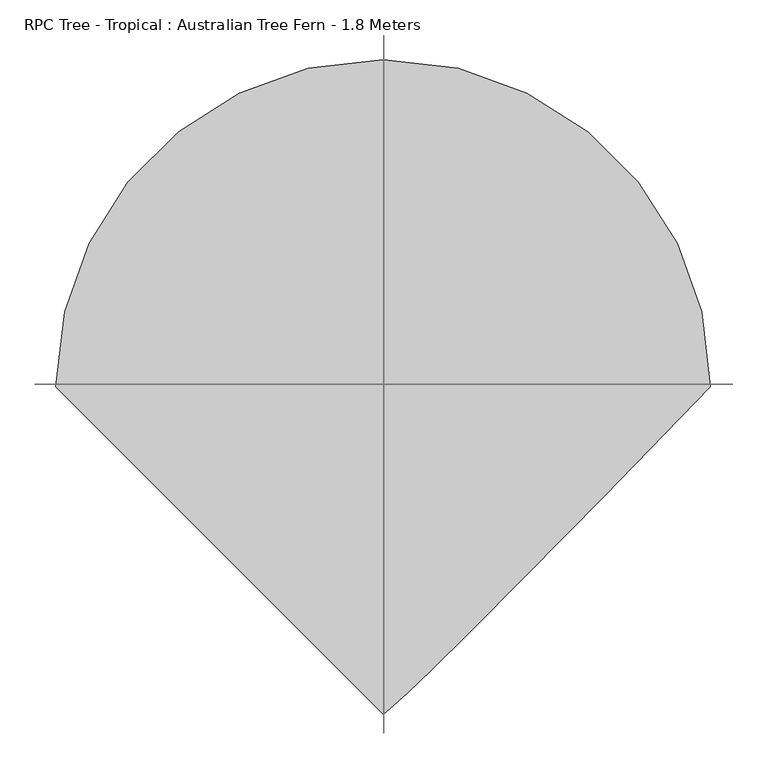
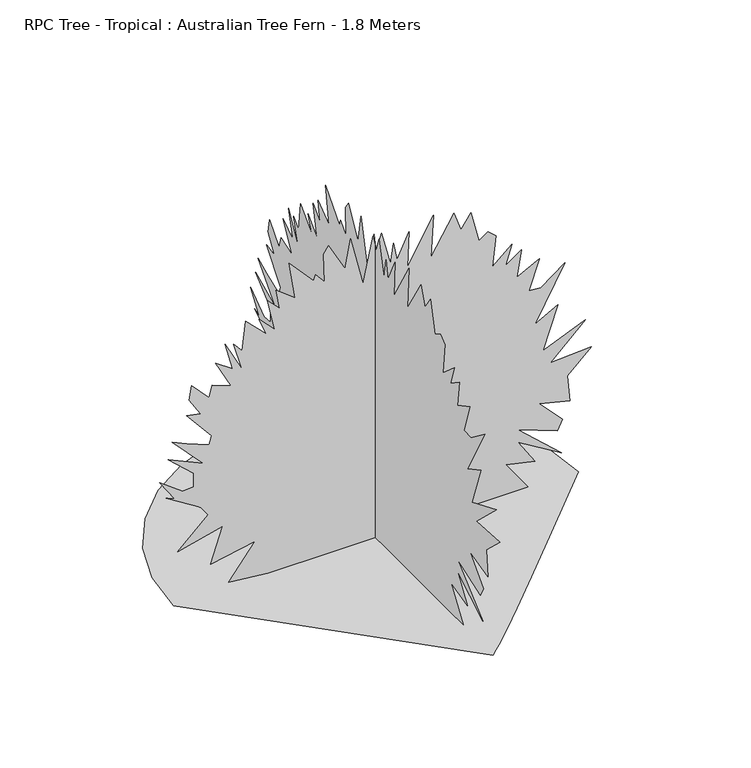
"""IFC4 building model written with IfcOpenShell, lengths in millimetres: geographic element geometry, RPC Tree - Tropical : Australian Tree Fern - 1.8 Meters."""

from ifc_helpers import new_model, si_unit, origin, place, context, project, spatial, triangles, source, transform, mapped, element, save


def rpc_tree_tropical_australian_tree_fern_1_8_meters_894294f9(model_context):
    return source(origin(), model_context, "Body", "Tessellation", [
        triangles([(-1121.4844528, 0.0, 0.0002091), (-1091.8312483, 257.014581, 0.0002091), (-1007.379063, 493.0422163, 0.0002091), (-874.8874409, 701.3197649, 0.0002091), (-701.1231199, 875.0840858, 0.0002091), (-492.845535, 1007.575708, 0.0002091), (-256.8179179, 1092.0278933, 0.0002091), (0.1967201, 1121.6810978, 0.0002091), (257.2112442, 1092.0278933, 0.0002091), (493.2388976, 1007.575708, 0.0002091), (701.5164099, 875.0840858, 0.0002091), (875.2807308, 701.3197649, 0.0002091), (1007.772353, 493.0422163, 0.0002091), (1092.2245382, 257.014581, 0.0002091), (1121.8777428, -9.81e-05, 0.0002091), (757.3559521, -373.9099531, 0.0002091), (487.118886, -649.203978, 0.0002091), (295.4501165, -842.3164639, 0.0002091), (166.6377574, -969.6837622, 0.0002091), (84.9673791, -1047.7439684, 0.0002091), (34.7249062, -1092.9297277, 0.0002091), (0.196524, -1121.6810978, 0.0002091), (-584.7020648, 9.9524755, 0.0280128), (-811.2515722, 9.9524573, 23.5990138), (-664.9373926, 9.9524755, 212.3913055), (-910.368124, 9.9524755, 165.1928965), (-844.2910526, 9.9524755, 363.42491), (-1094.439374, 9.9524755, 302.0672271), (-924.5263441, 9.9524948, 457.820202), (-967.0045652, 9.9524948, 519.177903), (-1155.7970387, 9.9524948, 637.1720089), (-1108.5994108, 9.9524948, 618.292638), (-1193.5540363, 9.9524948, 741.0079674), (-1066.121117, 9.9524948, 646.6127117), (-1004.7634523, 9.9524948, 651.3321184), (-1004.7634523, 9.9524948, 731.5673372), (-1146.3564085, 9.952513, 859.002146), (-952.8445284, 9.952513, 769.3262243), (-1122.7575583, 9.952513, 953.399291), (-1042.5223394, 9.952513, 915.6404039), (-919.8069374, 9.952513, 868.4427761), (-905.6469006, 9.952513, 915.6404039), (-1042.5223394, 9.952513, 1080.8322104), (-967.0045652, 9.952513, 1066.6740629), (-1028.3623026, 9.9525323, 1165.7887253), (-1014.2022657, 9.9525323, 1246.0258335), (-919.8069374, 9.9525323, 1142.1899477), (-900.9274939, 9.9525323, 1208.2670191), (-797.0915354, 9.9525323, 1170.508132), (-882.0480503, 9.9525323, 1330.9824211), (-787.652722, 9.9525323, 1264.9053497), (-830.1310158, 9.9525504, 1425.3776768), (-735.7356874, 9.9525323, 1246.0258335), (-782.9333879, 9.9525504, 1406.4983059), (-735.7356874, 9.9525323, 1354.5812714), (-716.8562439, 9.9525504, 1519.7729324), (-603.5815084, 9.9525504, 1406.4983059), (-641.3385424, 9.9525504, 1505.614785), (-556.3819911, 9.9525504, 1415.9388634), (-594.1408419, 9.9525504, 1595.2907066), (-528.0637705, 9.9525504, 1529.2136353), (-546.943214, 9.9525504, 1642.4884071), (-443.1072556, 9.9525504, 1562.2512989), (-476.146736, 9.9525697, 1774.6425499), (-339.2712971, 9.9525504, 1623.6088909), (-329.83252, 9.9525504, 1656.648444), (-279.7754919, 9.9525504, 1596.614463), (-284.4967516, 9.9525697, 1761.8062695), (-256.1691566, 9.9525697, 1800.0058273), (-164.5496218, 9.9525697, 1634.348933), (-134.8663864, 9.9525323, 1797.6189091), (-66.8546674, 9.9525323, 1511.5436382), (-8.8864392, 9.9525697, 1769.9232159), (9.9927528, 9.9525504, 1680.2472942), (38.3116059, 9.9525697, 1769.9232159), (85.5096334, 9.9525504, 1576.4113358), (104.3886955, 9.9525504, 1689.6861076), (123.2679392, 9.9525504, 1585.8501492), (189.3454011, 9.9525697, 1727.4448494), (179.9054977, 9.9525504, 1524.4943012), (326.2189688, 9.9525697, 1774.6425499), (312.0589319, 9.9525504, 1533.9331146), (439.4937043, 9.9525697, 1746.3243656), (477.2525914, 9.9525504, 1637.7690731), (533.8908857, 9.9525697, 1718.0042919), (576.3691432, 9.9525504, 1538.6524487), (628.2861414, 9.9525504, 1571.6918564), (670.7644352, 9.9525504, 1533.9331146), (651.8849916, 9.9525323, 1359.3006054), (760.4403568, 9.9525504, 1453.6958611), (722.6814697, 9.9525323, 1340.4212345), (812.3573914, 9.9525504, 1401.7788265), (788.7585411, 9.9525323, 1250.7453129), (911.4739431, 9.9525323, 1316.8223843), (854.8356125, 9.9525323, 1146.9092817), (920.9127565, 9.9525323, 1142.1899477), (1053.0668993, 9.9525323, 1241.3064995), (887.8750929, 9.952513, 939.2392542), (1015.3099016, 9.952513, 1010.0357323), (930.3533867, 9.952513, 769.3262243), (1166.3416712, 9.952513, 868.4427761), (972.8316078, 9.9524948, 684.3697094), (1199.3811516, 9.9524948, 698.5297462), (1067.2269361, 9.9524948, 575.8143442), (1081.386973, 9.9524755, 424.7807216), (911.4739431, 9.9524948, 467.2590154), (1038.9087519, 9.9524755, 330.3854296), (1010.5886055, 9.9524755, 273.7490065), (793.4779478, 9.9524755, 353.9842435), (1034.1874557, 9.9524755, 136.8741308), (793.4779478, 9.9524755, 283.1877836), (887.8750929, 9.9524755, 136.8741308), (727.4008764, 9.9524755, 174.6324366), (850.2137289, 9.9524755, 0.0285496), (14.7125365, 9.9524573, 9.11e-05), (2.9132547, 597.5662868, 0.0279397), (2.913236, 824.1176474, 23.5990138), (2.9132547, 677.8033951, 212.3913055), (2.9132547, 923.2323097, 165.1928965), (2.9132547, 857.1552383, 363.42491), (2.9132547, 1107.3054491, 302.0672271), (2.9132547, 937.3923466, 457.820202), (2.9132547, 979.8706404, 519.177903), (2.9132735, 1168.6612244, 637.1720089), (2.9132735, 1121.4635965, 618.292638), (2.9132735, 1206.4201115, 741.0079674), (2.9132735, 1078.9853027, 646.6127117), (2.9132735, 1017.6295275, 651.3321184), (2.9132735, 1017.6295275, 731.5673372), (2.9132735, 1159.2224836, 859.002146), (2.9132735, 965.7106035, 769.3262243), (2.9132735, 1135.6236334, 953.399291), (2.9132735, 1055.3865252, 915.6404039), (2.9132735, 932.6730125, 868.4427761), (2.9132735, 918.5129757, 915.6404039), (2.9132735, 1055.3865252, 1080.8322104), (2.9132735, 979.8706404, 1066.6740629), (2.9132735, 1041.2283051, 1165.7887253), (2.9132922, 1027.0682682, 1246.0258335), (2.9132735, 932.6730125, 1142.1899477), (2.9132735, 913.793569, 1208.2670191), (2.9132735, 809.9576105, 1170.5100214), (2.9132922, 894.9141254, 1330.9824211), (2.9132735, 800.5187971, 1264.9053497), (2.9132922, 842.9970909, 1425.3776768), (2.9132735, 748.5998732, 1246.0258335), (2.9132922, 795.7975737, 1406.4983059), (2.9132735, 748.5998732, 1354.5812714), (2.9132922, 729.722319, 1519.7729324), (2.9132735, 616.4457304, 1406.4983059), (2.9132922, 654.2046175, 1505.614785), (2.9132735, 569.2480662, 1415.9388634), (2.9132922, 607.0069533, 1595.2907066), (2.9132922, 540.9298456, 1529.2136353), (2.9132922, 559.8092892, 1642.4884071), (2.9132922, 455.9733307, 1562.2512989), (2.9132922, 489.010958, 1774.6425499), (2.9132922, 352.1373722, 1623.6088909), (2.9132922, 342.6985951, 1656.648444), (2.9132922, 292.641567, 1596.614463), (2.9132922, 297.3609555, 1761.8062695), (2.9132922, 269.0352317, 1800.0058273), (2.9132922, 177.4153154, 1634.348933), (2.9132547, 147.7320982, 1797.6189091), (2.9132547, 79.72057, 1511.5455276), (2.9132922, 21.7521334, 1769.9232159), (2.9132735, 2.872978, 1680.2472942), (2.9132922, -25.4458941, 1769.9232159), (2.9132735, -72.6439216, 1576.4113358), (2.9132735, -91.5229837, 1689.6861076), (2.9132735, -110.4020457, 1585.8518932), (2.9132735, -176.4793078, 1727.4448494), (2.9132735, -167.0397859, 1524.4943012), (2.9132735, -313.3528936, 1774.6425499), (2.9132735, -299.1947099, 1533.9331146), (2.9132735, -426.6276292, 1746.3243656), (2.9132735, -464.3864799, 1637.7690731), (2.9132735, -521.0248106, 1718.0061813), (2.9132735, -563.5030681, 1538.6524487), (2.9132735, -615.4200663, 1571.6918564), (2.9132735, -657.8983601, 1533.9331146), (2.9132547, -639.0189165, 1359.3006054), (2.9132547, -747.5742817, 1453.6958611), (2.9132547, -709.8153946, 1340.4212345), (2.9132547, -799.4913162, 1401.7788265), (2.9132547, -775.892466, 1250.7453129), (2.9132547, -898.607868, 1316.8223843), (2.9132547, -841.96961, 1146.9092817), (2.9132547, -908.0466814, 1142.1899477), (2.9132547, -1040.2008242, 1241.3064995), (2.9132547, -875.0090904, 939.2392542), (2.9132547, -1002.4438265, 1010.0357323), (2.913236, -917.4873116, 769.3262243), (2.913236, -1153.4774855, 868.4427761), (2.913236, -959.9656054, 684.3697094), (2.913236, -1186.5150764, 698.5297462), (2.913236, -1054.360861, 575.8143442), (2.913236, -1068.5208979, 424.7807216), (2.913236, -898.607868, 467.2590154), (2.9132173, -1026.0426767, 330.3854296), (2.9132173, -997.7244198, 273.7490065), (2.913236, -780.6137621, 353.9842435), (2.9132173, -1021.32327, 136.8739401), (2.913236, -780.6137621, 283.1877836), (2.9132173, -875.0090904, 136.8739401), (2.9132173, -714.5366907, 174.6324366), (2.913236, -837.3476538, 0.0284335), (2.913236, -1.8467684, 0.0)], [[22, 21, 1], [21, 20, 1], [20, 19, 1], [19, 18, 1], [18, 17, 1], [1, 17, 2], [2, 17, 3], [3, 17, 4], [17, 16, 4], [4, 16, 5], [5, 16, 6], [6, 16, 7], [7, 16, 8], [8, 16, 9], [9, 16, 10], [10, 16, 11], [11, 16, 12], [16, 15, 12], [15, 14, 12], [14, 13, 12], [31, 30, 32], [110, 109, 111], [52, 51, 53], [37, 36, 38], [33, 32, 34], [77, 76, 78], [101, 100, 102], [39, 38, 40], [79, 78, 80], [58, 57, 59], [71, 70, 72], [97, 96, 98], [73, 72, 74], [54, 53, 55], [81, 80, 82], [50, 49, 51], [28, 27, 29], [90, 89, 91], [75, 74, 76], [60, 59, 61], [64, 63, 65], [40, 38, 41], [103, 102, 104], [43, 42, 44], [99, 98, 100], [62, 61, 63], [94, 93, 95], [112, 111, 113], [92, 91, 93], [85, 84, 86], [83, 82, 84], [56, 55, 57], [46, 45, 47], [45, 44, 47], [114, 113, 115], [66, 65, 67], [24, 23, 25], [74, 72, 76], [26, 25, 27], [69, 68, 70], [68, 67, 70], [32, 30, 34], [34, 30, 35], [105, 104, 106], [51, 49, 53], [104, 102, 106], [96, 95, 98], [48, 47, 49], [108, 107, 109], [107, 106, 109], [84, 82, 86], [87, 86, 88], [88, 86, 89], [70, 67, 72], [23, 115, 25], [55, 53, 57], [86, 82, 89], [78, 76, 80], [65, 63, 67], [61, 59, 63], [44, 42, 47], [47, 42, 49], [36, 35, 38], [76, 72, 80], [113, 111, 115], [111, 109, 115], [102, 100, 106], [106, 100, 109], [109, 100, 115], [100, 98, 115], [115, 98, 25], [98, 95, 25], [95, 93, 25], [93, 91, 25], [91, 89, 25], [89, 82, 25], [82, 80, 25], [80, 72, 25], [25, 72, 27], [27, 72, 29], [72, 67, 29], [67, 63, 29], [63, 59, 29], [29, 59, 30], [30, 59, 35], [35, 59, 38], [38, 59, 41], [41, 59, 42], [42, 59, 49], [49, 59, 53], [53, 59, 57], [124, 123, 125], [203, 202, 204], [145, 144, 146], [130, 129, 131], [126, 125, 127], [170, 169, 171], [194, 193, 195], [132, 131, 133], [172, 171, 173], [151, 150, 152], [164, 163, 165], [190, 189, 191], [166, 165, 167], [147, 146, 148], [174, 173, 175], [143, 142, 144], [121, 120, 122], [183, 182, 184], [168, 167, 169], [153, 152, 154], [157, 156, 158], [133, 131, 134], [196, 195, 197], [136, 135, 137], [192, 191, 193], [155, 154, 156], [187, 186, 188], [205, 204, 206], [185, 184, 186], [178, 177, 179], [176, 175, 177], [149, 148, 150], [139, 138, 140], [138, 137, 140], [207, 206, 208], [159, 158, 160], [117, 116, 118], [167, 165, 169], [119, 118, 120], [162, 161, 163], [161, 160, 163], [125, 123, 127], [127, 123, 128], [198, 197, 199], [144, 142, 146], [197, 195, 199], [189, 188, 191], [141, 140, 142], [201, 200, 202], [200, 199, 202], [177, 175, 179], [180, 179, 181], [181, 179, 182], [163, 160, 165], [116, 208, 118], [148, 146, 150], [179, 175, 182], [171, 169, 173], [158, 156, 160], [154, 152, 156], [137, 135, 140], [140, 135, 142], [129, 128, 131], [169, 165, 173], [206, 204, 208], [204, 202, 208], [195, 193, 199], [199, 193, 202], [202, 193, 208], [193, 191, 208], [208, 191, 118], [191, 188, 118], [188, 186, 118], [186, 184, 118], [184, 182, 118], [182, 175, 118], [175, 173, 118], [173, 165, 118], [118, 165, 120], [120, 165, 122], [165, 160, 122], [160, 156, 122], [156, 152, 122], [122, 152, 123], [123, 152, 128], [128, 152, 131], [131, 152, 134], [134, 152, 135], [135, 152, 142], [142, 152, 146], [146, 152, 150]], closed=False),
    ])


if __name__ == "__main__":
    model = new_model("IFC4")
    model_context = context("Model", 3, world=origin())
    ifc_project = project(units=[si_unit("LENGTHUNIT", "METRE", prefix="MILLI")], contexts=[model_context])
    site = spatial("IfcSite", under=ifc_project)
    building = spatial("IfcBuilding", under=site)
    placement = place(None, origin())
    rpc_tree_tropical_australian_tree_fern_1_8_meters_shape = rpc_tree_tropical_australian_tree_fern_1_8_meters_894294f9(model_context)
    element("IfcGeographicElement", 1, ObjectType="RPC Tree - Tropical : Australian Tree Fern - 1.8 Meters", at=placement, inside=building, context=model_context, shape_type="MappedRepresentation", body=[
        mapped(rpc_tree_tropical_australian_tree_fern_1_8_meters_shape, transform((0.0, 0.0, 0.0), x_axis=(1.0, 0.0, 0.0), y_axis=(0.0, 1.0, 0.0), z_axis=(0.0, 0.0, 1.0))),
    ])
    save(model, "model.ifc")

# Revit data of these elements
# Type "RPC Tree - Tropical : Australian Tree Fern - 1.8 Meters"
#   built-in parameter 1005195 = "RPC-16-G2F6-877X-GLVN-N000-ST1L-LVER-AU"
#   Type Comments = "Australian Tree Fern"
#   Height = 1800 mm
#   Plan Symbol = element 242927
#   Description = (empty or 0)
